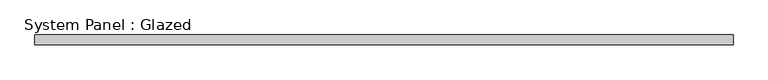
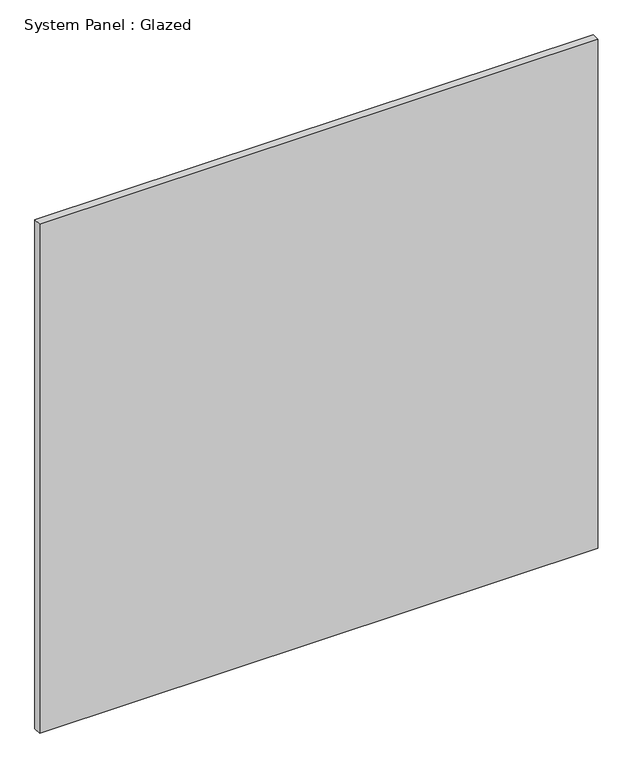
"""IFC4 building model written with IfcOpenShell, lengths in millimetres: plate geometry, System Panel : Glazed."""

from ifc_helpers import new_model, si_unit, origin, origin_with_axes, place, context, project, spatial, polyline, outline, extrude, source, transform, mapped, element, save


def system_panel_glazed_67319d03(model_context):
    return source(origin(), model_context, "Body", "SweptSolid", [
        extrude(outline(polyline([(877.5000002, 24.5), (-877.5000002, 24.5), (-877.5000002, 49.5), (877.5000002, 49.5), (877.5000002, 24.5)])), origin_with_axes(), (0.0, 0.0, 1.0), 1690.2939092),
    ])


if __name__ == "__main__":
    model = new_model("IFC4")
    model_context = context("Model", 3, world=origin())
    ifc_project = project(units=[si_unit("LENGTHUNIT", "METRE", prefix="MILLI")], contexts=[model_context])
    site = spatial("IfcSite", under=ifc_project)
    building = spatial("IfcBuilding", under=site)
    placement = place(None, origin())
    system_panel_glazed_shape = system_panel_glazed_67319d03(model_context)
    element("IfcPlate", 1, ObjectType="System Panel : Glazed", at=placement, inside=building, context=model_context, shape_type="MappedRepresentation", body=[
        mapped(system_panel_glazed_shape, transform((0.0, 0.0, 0.0), x_axis=(1.0, 0.0, 0.0), y_axis=(0.0, 1.0, 0.0), z_axis=(0.0, 0.0, 1.0))),
    ])
    save(model, "model.ifc")

# Revit data of these elements
# Element 1 (IfcPlate, "System Panel : Glazed")
#   Materials on its faces: "Glass"
# Materials
#   "Glass": class "Glass", colour RGB 218 227 224, transparency 0.85, Description = "Soda Lime Glass", Cost = 0
